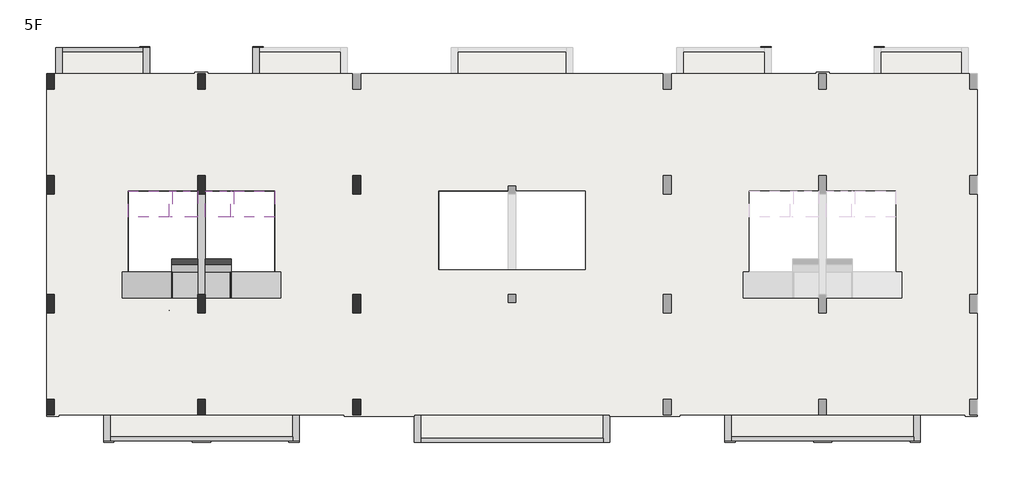
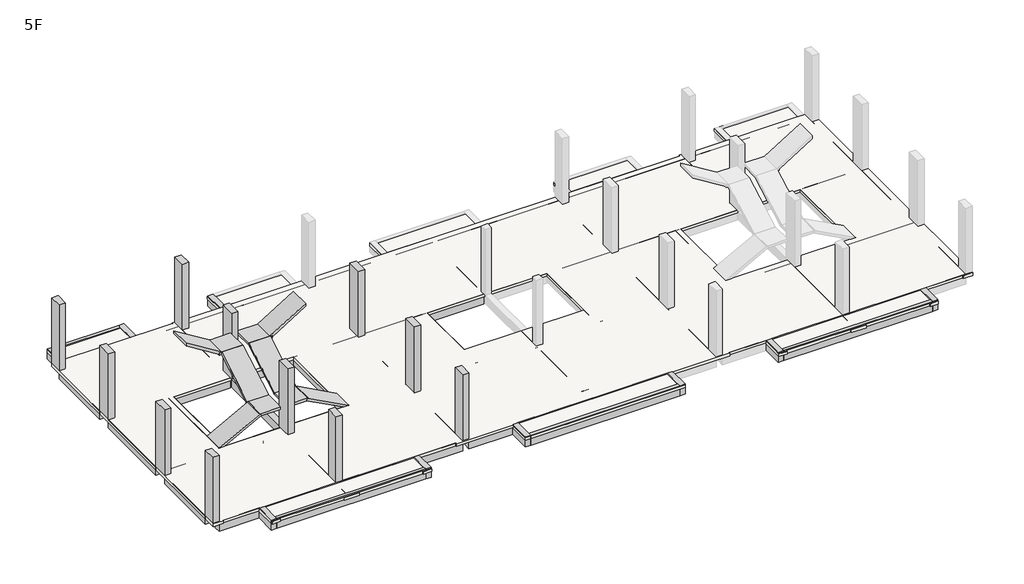
# One storey, part 1 of 2: 48 beams, 11 columns, 2 slabs.
"""IFC4 building model written with IfcOpenShell, lengths in millimetres."""

from ifc_helpers import new_model, si_unit, frame, origin, place, context, project, spatial, polyline, outline, extrude, faceted_brep, element, save

model = new_model("IFC4")

# Units and contexts
model_context = context("Model", 3, world=origin())
ifc_project = project(units=[si_unit("LENGTHUNIT", "METRE", prefix="MILLI")], contexts=[model_context])

# Site, building, storey
site = spatial("IfcSite", under=ifc_project)
building = spatial("IfcBuilding", under=site)
storey = spatial("IfcBuildingStorey", under=building, Name="5F", Elevation=13930.0)

# Beams
placement = place(None, origin())
element("IfcBeam", 1, ObjectType="M_Concrete-Rectangular Beam : 1000x120", at=placement, inside=storey, context=model_context, shape_type="Brep", body=[
    faceted_brep([(4730.4772067, 5424.9999998, 14980.0), (4730.4772067, 4424.9999998, 14980.0), (4787.1330577, 4424.9999998, 14874.2166623), (4787.1330577, 5424.9999998, 14874.2166623), (4700.0000007, 5424.9999998, 14963.6768996), (2770.0, 5424.9999998, 13930.0), (2770.0, 4424.9999998, 13930.0), (4700.0000007, 4424.9999998, 14963.6768996), (3024.1661582, 4424.9999998, 13930.0), (4760.5888269, 4424.9999998, 14860.0), (3024.1661582, 4449.9999998, 13930.0), (3020.0, 4449.9999998, 13927.7686728), (3020.0, 5424.9999998, 13927.7686728), (4760.5888269, 5424.9999998, 14860.0), (3020.0, 5424.9999998, 13930.0), (3020.0, 4449.9999998, 13930.0)], [[[0, 1, 2, 3]], [[1, 0, 4, 5, 6, 7]], [[2, 1, 7, 6, 8, 9]], [[3, 2, 9, 8, 10, 11, 12, 13]], [[0, 3, 13, 12, 14, 5, 4]], [[5, 14, 15, 10, 8, 6]], [[14, 12, 11, 15]], [[10, 15, 11]]]),
])
element("IfcBeam", 2, ObjectType="M_Concrete-Rectangular Beam : 1000x120", at=placement, inside=storey, context=model_context, shape_type="Brep", body=[
    faceted_brep([(4700.0000007, 7550.0000002, 16180.0), (5700.0000007, 7550.0000002, 16180.0), (5700.0000007, 7609.0063595, 16075.5095719), (4700.0000007, 7609.0063595, 16075.5095719), (4700.0000007, 5424.9999998, 14980.0), (4700.0000007, 5484.0063591, 14875.5095719), (5700.0000007, 5484.0063591, 14875.5095719), (5700.0000007, 5424.9999998, 14980.0), (5700.0000007, 5524.9999998, 14898.6589219), (5700.0000007, 7581.5414925, 16060.0), (4700.0000007, 5524.9999998, 14898.6589219), (4700.0000007, 7581.5414925, 16060.0)], [[[0, 1, 2, 3]], [[4, 5, 6, 7]], [[1, 0, 4, 7]], [[2, 1, 7, 6, 8, 9]], [[3, 2, 9, 8, 6, 5, 10, 11]], [[0, 3, 11, 10, 5, 4]]]),
])
element("IfcBeam", 3, ObjectType="M_Concrete-Rectangular Beam : 1000x120", at=placement, inside=storey, context=model_context, shape_type="Brep", body=[
    faceted_brep([(4600.0000007, 7550.0000002, 16180.0), (4600.0000007, 8550.0000002, 16180.0), (4600.0000007, 8550.0000002, 16060.0), (4600.0000007, 7550.0000002, 16060.0), (5700.0000007, 8550.0000002, 16060.0), (5700.0000007, 8550.0000002, 16180.0), (5700.0000007, 7550.0000002, 16180.0), (5700.0000007, 7609.0063595, 16075.5095719), (5700.0000007, 7581.5414925, 16060.0), (4700.0000007, 7550.0000002, 16180.0), (4700.0000007, 7581.5414925, 16060.0), (4700.0000007, 7550.0000002, 16060.0), (4700.0000007, 7609.0063595, 16075.5095719)], [[[0, 1, 2, 3]], [[4, 5, 6, 7, 8]], [[1, 0, 9, 6, 5]], [[2, 1, 5, 4]], [[3, 2, 4, 8, 10, 11]], [[0, 3, 11, 9]], [[12, 7, 6, 9]], [[7, 12, 10, 8]], [[12, 9, 11, 10]]]),
])
element("IfcBeam", 4, ObjectType="M_Concrete-Rectangular Beam : 1000x120", at=placement, inside=storey, context=model_context, shape_type="Brep", body=[
    faceted_brep([(3019.99996, 7549.9999993, 17230.0), (4715.7503089, 7549.9999993, 16180.0), (4715.7503089, 8549.9999993, 16180.0), (3019.99996, 8549.9999993, 17230.0), (4600.0000007, 8549.9999993, 16180.0), (4600.0000007, 8549.9999993, 16110.5302519), (3020.0, 8549.9999993, 17088.8582245), (4600.0000007, 7549.9999993, 16110.5302519), (3020.0, 7549.9999993, 17088.8582245), (4600.0000007, 7549.9999993, 16180.0), (4700.0000007, 7549.9999993, 16180.0)], [[[0, 1, 2, 3]], [[3, 2, 4, 5, 6]], [[5, 7, 8, 6]], [[1, 0, 8, 7, 9, 10]], [[4, 9, 7, 5]], [[9, 4, 2, 1, 10]], [[0, 3, 6, 8]]]),
])
element("IfcBeam", 5, ObjectType="M_Concrete-Rectangular Beam : 1000x120", at=placement, inside=storey, context=model_context, shape_type="Brep", body=[
    faceted_brep([(5700.0000007, 5524.9999998, 14860.0), (4700.0000007, 5524.9999998, 14860.0), (4700.0000007, 5524.9999998, 14898.6589219), (5700.0000007, 5524.9999998, 14898.6589219), (5700.0000007, 4424.9999998, 14860.0), (5700.0000007, 4424.9999998, 14980.0), (4730.4772067, 4424.9999998, 14980.0), (4787.1330577, 4424.9999998, 14874.2166623), (4760.5888269, 4424.9999998, 14860.0), (5700.0000007, 5424.9999998, 14980.0), (4700.0000007, 5424.9999998, 14980.0), (4700.0000007, 4424.9999998, 14980.0), (5700.0000007, 5484.0063591, 14875.5095719), (4760.5888269, 5424.9999998, 14860.0), (4700.0000007, 5424.9999998, 14860.0), (4700.0000007, 4424.9999998, 14963.6768996), (4700.0000007, 5484.0063591, 14875.5095719), (4700.0000007, 5424.9999998, 14963.6768996), (4730.4772067, 5424.9999998, 14980.0), (4787.1330577, 5424.9999998, 14874.2166623)], [[[0, 1, 2, 3]], [[4, 5, 6, 7, 8]], [[6, 5, 9, 10, 11]], [[5, 4, 0, 3, 12, 9]], [[1, 0, 4, 8, 13, 14]], [[15, 11, 10, 16, 2, 1, 14, 17]], [[6, 18, 19, 7]], [[18, 6, 15, 17]], [[7, 19, 13, 8]], [[19, 18, 17, 14, 13]], [[11, 15, 6]], [[12, 16, 10, 9]], [[16, 12, 3, 2]]]),
])
element("IfcBeam", 6, ObjectType="M_Concrete-Rectangular Beam : 1000x120", at=placement, inside=storey, context=model_context, shape_type="Brep", body=[
    faceted_brep([(6969.5227948, 4424.9999998, 14980.0), (6969.5227948, 5424.9999998, 14980.0), (6912.8669437, 5424.9999998, 14874.2166623), (6912.8669437, 4424.9999998, 14874.2166623), (7000.0000007, 4424.9999998, 14963.6768996), (8930.0000014, 4424.9999998, 13930.0), (8930.0000014, 5424.9999998, 13930.0), (7000.0000007, 5424.9999998, 14963.6768996), (6939.4111745, 4424.9999998, 14860.0), (8675.8338433, 4424.9999998, 13930.0), (6939.4111745, 5424.9999998, 14860.0), (8680.0, 5424.9999998, 13927.7686736), (8680.0, 4449.9999998, 13927.7686736), (8675.8338433, 4449.9999998, 13930.0), (8680.0, 5424.9999998, 13930.0), (8680.0, 4449.9999998, 13930.0)], [[[0, 1, 2, 3]], [[1, 0, 4, 5, 6, 7]], [[0, 3, 8, 9, 5, 4]], [[3, 2, 10, 11, 12, 13, 9, 8]], [[2, 1, 7, 6, 14, 11, 10]], [[9, 13, 15, 14, 6, 5]], [[11, 14, 15, 12]], [[15, 13, 12]]]),
])
element("IfcBeam", 7, ObjectType="M_Concrete-Rectangular Beam : 1000x120", at=placement, inside=storey, context=model_context, shape_type="Brep", body=[
    faceted_brep([(7000.0000007, 7550.0000002, 16180.0), (7000.0000007, 7609.0063595, 16075.5095719), (6000.0000007, 7609.0063595, 16075.5095719), (6000.0000007, 7550.0000002, 16180.0), (7000.0000007, 5424.9999998, 14980.0), (6000.0000007, 5424.9999998, 14980.0), (6000.0000007, 5484.0063591, 14875.5095719), (7000.0000007, 5484.0063591, 14875.5095719), (6000.0000007, 7581.5414925, 16060.0), (6000.0000007, 5524.9999998, 14898.6589219), (7000.0000007, 7581.5414925, 16060.0), (7000.0000007, 5524.9999998, 14898.6589219)], [[[0, 1, 2, 3]], [[4, 5, 6, 7]], [[3, 5, 4, 0]], [[2, 8, 9, 6, 5, 3]], [[1, 10, 11, 7, 6, 9, 8, 2]], [[0, 4, 7, 11, 10, 1]]]),
])
element("IfcBeam", 8, ObjectType="M_Concrete-Rectangular Beam : 1000x120", at=placement, inside=storey, context=model_context, shape_type="Brep", body=[
    faceted_brep([(7100.0000007, 8550.0000002, 16180.0), (7100.0000007, 7550.0000002, 16180.0), (7100.0000007, 7550.0000002, 16060.0), (7100.0000007, 8550.0000002, 16060.0), (6000.0000007, 8550.0000002, 16180.0), (6000.0000007, 8550.0000002, 16060.0), (6000.0000007, 7581.5414925, 16060.0), (6000.0000007, 7609.0063595, 16075.5095719), (6000.0000007, 7550.0000002, 16180.0), (7000.0000007, 7550.0000002, 16180.0), (7000.0000007, 7550.0000002, 16060.0), (7000.0000007, 7581.5414925, 16060.0), (7000.0000007, 7609.0063595, 16075.5095719)], [[[0, 1, 2, 3]], [[4, 5, 6, 7, 8]], [[1, 0, 4, 8, 9]], [[0, 3, 5, 4]], [[3, 2, 10, 11, 6, 5]], [[2, 1, 9, 10]], [[12, 9, 8, 7]], [[12, 7, 6, 11]], [[9, 12, 11, 10]]]),
])
element("IfcBeam", 9, ObjectType="M_Concrete-Rectangular Beam : 1000x120", at=placement, inside=storey, context=model_context, shape_type="Brep", body=[
    faceted_brep([(6984.2496926, 7549.9999993, 16180.0), (8680.0000414, 7549.9999993, 17230.0), (8680.0, 8549.9999993, 17229.9999744), (6984.2496926, 8549.9999993, 16180.0), (8680.0, 8549.9999993, 17088.8582236), (7100.0000007, 8549.9999993, 16110.5302519), (7100.0000007, 8549.9999993, 16180.0), (7100.0000007, 7549.9999993, 16110.5302519), (8680.0, 7549.9999993, 17088.8582236), (7000.0000007, 7549.9999993, 16180.0), (7100.0000007, 7549.9999993, 16180.0)], [[[0, 1, 2, 3]], [[3, 2, 4, 5, 6]], [[7, 5, 4, 8]], [[1, 0, 9, 10, 7, 8]], [[10, 6, 5, 7]], [[6, 10, 9, 0, 3]], [[2, 1, 8, 4]]]),
])
element("IfcBeam", 10, ObjectType="M_Concrete-Rectangular Beam : 1000x120", at=placement, inside=storey, context=model_context, shape_type="Brep", body=[
    faceted_brep([(7000.0000007, 5524.9999998, 14860.0), (6000.0000007, 5524.9999998, 14860.0), (6000.0000007, 5524.9999998, 14898.6589219), (7000.0000007, 5524.9999998, 14898.6589219), (6000.0000007, 4424.9999998, 14980.0), (6000.0000007, 4424.9999998, 14860.0), (6939.4111745, 4424.9999998, 14860.0), (6912.8669437, 4424.9999998, 14874.2166623), (6969.5227948, 4424.9999998, 14980.0), (7000.0000007, 4424.9999998, 14980.0), (7000.0000007, 5424.9999998, 14980.0), (6000.0000007, 5424.9999998, 14980.0), (6000.0000007, 5484.0063591, 14875.5095719), (7000.0000007, 5424.9999998, 14860.0), (6939.4111745, 5424.9999998, 14860.0), (7000.0000007, 4424.9999998, 14963.6768996), (7000.0000007, 5424.9999998, 14963.6768996), (7000.0000007, 5484.0063591, 14875.5095719), (6969.5227948, 5424.9999998, 14980.0), (6912.8669437, 5424.9999998, 14874.2166623)], [[[0, 1, 2, 3]], [[4, 5, 6, 7, 8]], [[8, 9, 10, 11, 4]], [[5, 4, 11, 12, 2, 1]], [[1, 0, 13, 14, 6, 5]], [[9, 15, 16, 13, 0, 3, 17, 10]], [[18, 8, 7, 19]], [[8, 18, 16, 15]], [[19, 7, 6, 14]], [[18, 19, 14, 13, 16]], [[15, 9, 8]], [[17, 12, 11, 10]], [[12, 17, 3, 2]]]),
])
element("IfcBeam", 11, ObjectType="M_Concrete-Rectangular Beam : 150x500", at=placement, inside=storey, context=model_context, shape_type="SweptSolid", body=[
    extrude(outline(polyline([(2320.0000398, -1099.9999999), (2320.0000398, -949.9999999), (9380.0000399, -949.9999999), (9380.0000399, -1099.9999999), (2320.0000398, -1099.9999999)])), frame((0.0, 0.0, 13430.0), z_axis=(0.0, 0.0, 1.0), x_axis=(1.0, 0.0, 0.0)), (0.0, 0.0, 1.0), 500.0),
])
element("IfcBeam", 12, ObjectType="M_Concrete-Rectangular Beam : 150x500", at=placement, inside=storey, context=model_context, shape_type="SweptSolid", body=[
    extrude(outline(polyline([(26320.012858, -1100.2407813), (26320.012858, -950.2407813), (33380.0128581, -950.2407813), (33380.0128581, -1100.2407813), (26320.012858, -1100.2407813)])), frame((0.0, 0.0, 13430.0), z_axis=(0.0, 0.0, 1.0), x_axis=(1.0, 0.0, 0.0)), (0.0, 0.0, 1.0), 500.0),
])
element("IfcBeam", 13, ObjectType="M_Concrete-Rectangular Beam : 150x500", at=placement, inside=storey, context=model_context, shape_type="SweptSolid", body=[
    extrude(outline(polyline([(14320.0998335, -1150.2407813), (14320.0998335, -1000.2407813), (21380.0998336, -1000.2407813), (21380.0998336, -1150.2407813), (14320.0998335, -1150.2407813)])), frame((0.0, 0.0, 13430.0), z_axis=(0.0, 0.0, 1.0), x_axis=(1.0, 0.0, 0.0)), (0.0, 0.0, 1.0), 500.0),
])
element("IfcBeam", 14, ObjectType="M_Concrete-Rectangular Beam : 150x500", at=placement, inside=storey, context=model_context, shape_type="SweptSolid", body=[
    extrude(outline(polyline([(3609.9999642, 14100.0000002), (3609.9999642, 13950.0000002), (475.0000398, 13950.0000002), (475.0000398, 14100.0000002), (3609.9999642, 14100.0000002)])), frame((0.0, 0.0, 13430.0), z_axis=(0.0, 0.0, 1.0), x_axis=(1.0, 0.0, 0.0)), (0.0, 0.0, 1.0), 500.0),
])
element("IfcBeam", 15, ObjectType="M_Concrete-Rectangular Beam : 250x400", at=placement, inside=storey, context=model_context, shape_type="Brep", body=[
    faceted_brep([(8930.0, 8549.9999993, 13930.0), (8680.0, 8549.9999993, 13930.0), (8680.0, 5424.9999998, 13930.0), (8680.0, 4449.9999998, 13930.0), (8930.0, 4449.9999998, 13930.0), (8680.0, 8549.9999993, 13788.8582236), (8680.0, 8549.9999993, 13530.0), (8680.0, 4449.9999998, 13530.0), (8680.0, 4449.9999998, 13927.7686736), (8930.0, 8549.9999993, 13530.0), (8930.0, 4449.9999998, 13530.0)], [[[0, 1, 2, 3, 4]], [[1, 5, 6, 7, 8, 3, 2]], [[6, 9, 10, 7]], [[9, 0, 4, 10]], [[1, 0, 9, 6, 5]], [[4, 3, 8, 7, 10]]]),
])
element("IfcBeam", 16, ObjectType="M_Concrete-Rectangular Beam : 250x400", at=placement, inside=storey, context=model_context, shape_type="Brep", body=[
    faceted_brep([(15020.0000057, 8549.9999993, 13930.0), (14770.0000057, 8549.9999993, 13930.0), (14770.0000057, 4449.9999998, 13930.0), (15020.0000057, 4449.9999998, 13930.0), (15020.0000057, 8549.9999993, 13530.0), (15020.0000057, 8549.9999993, 13788.8582241), (15020.0000057, 4449.9999998, 13530.0), (14770.0000057, 8549.9999993, 13530.0), (14770.0000057, 4449.9999998, 13530.0)], [[[0, 1, 2, 3]], [[4, 5, 0, 3, 6]], [[7, 4, 6, 8]], [[1, 7, 8, 2]], [[1, 0, 5, 4, 7]], [[3, 2, 8, 6]]]),
])
element("IfcBeam", 17, ObjectType="M_Concrete-Rectangular Beam : 250x400", at=placement, inside=storey, context=model_context, shape_type="Brep", body=[
    faceted_brep([(3020.0, 8549.9999993, 13930.0), (2770.0, 8549.9999993, 13930.0), (2770.0, 4449.9999998, 13930.0), (3020.0, 4449.9999998, 13930.0), (3020.0, 5424.9999998, 13930.0), (3020.0, 8549.9999993, 13530.0), (3020.0, 8549.9999993, 13788.8582245), (3020.0, 4449.9999998, 13927.7686728), (3020.0, 4449.9999998, 13530.0), (2770.0, 8549.9999993, 13530.0), (2770.0, 4449.9999998, 13530.0)], [[[0, 1, 2, 3, 4]], [[5, 6, 0, 4, 3, 7, 8]], [[9, 5, 8, 10]], [[1, 9, 10, 2]], [[1, 0, 6, 5, 9]], [[3, 2, 10, 8, 7]]]),
])
element("IfcBeam", 18, ObjectType="M_Concrete-Rectangular Beam : 250x500", at=placement, inside=storey, context=model_context, shape_type="Brep", body=[
    faceted_brep([(225.0000398, 13101.5853605, 13930.0), (225.0000398, 13101.5853605, 13430.0), (475.0000398, 13101.5853605, 13430.0), (475.0000398, 13101.5853605, 13930.0), (475.0000398, 13950.0000002, 13930.0), (475.0000398, 14100.0000002, 13930.0), (225.0000398, 14100.0000002, 13930.0), (475.0000398, 13950.0000002, 13430.0), (475.0000398, 14100.0000002, 13430.0), (225.0000398, 14100.0000002, 13430.0)], [[[0, 1, 2, 3]], [[0, 3, 4, 5, 6]], [[3, 2, 7, 8, 5, 4]], [[2, 1, 9, 8, 7]], [[1, 0, 6, 9]], [[6, 5, 8, 9]]]),
])
element("IfcBeam", 19, ObjectType="M_Concrete-Rectangular Beam : 250x500", at=placement, inside=storey, context=model_context, shape_type="Brep", body=[
    faceted_brep([(2070.0000398, -1099.9999999, 13930.0), (2320.0000398, -1099.9999999, 13930.0), (2320.0000398, -949.9999999, 13930.0), (2320.0000398, -100.0000007, 13930.0), (2070.0000398, -100.0000007, 13930.0), (2320.0000398, -1099.9999999, 13430.0), (2320.0000398, -949.9999999, 13430.0), (2320.0000398, -100.0000007, 13430.0), (2070.0000398, -1099.9999999, 13430.0), (2070.0000398, -100.0000007, 13430.0)], [[[0, 1, 2, 3, 4]], [[1, 5, 6, 7, 3, 2]], [[5, 8, 9, 7, 6]], [[8, 0, 4, 9]], [[4, 3, 7, 9]], [[1, 0, 8, 5]]]),
])
element("IfcBeam", 20, ObjectType="M_Concrete-Rectangular Beam : 250x500", at=placement, inside=storey, context=model_context, shape_type="Brep", body=[
    faceted_brep([(9380.0000399, -1099.9999999, 13930.0), (9630.0000399, -1099.9999999, 13930.0), (9630.0000399, -100.0000007, 13930.0), (9380.0000399, -100.0000007, 13930.0), (9380.0000399, -949.9999999, 13930.0), (9380.0000399, -1099.9999999, 13430.0), (9380.0000399, -100.0000007, 13430.0), (9380.0000399, -949.9999999, 13430.0), (9630.0000399, -1099.9999999, 13430.0), (9630.0000399, -100.0000007, 13430.0)], [[[0, 1, 2, 3, 4]], [[5, 0, 4, 3, 6, 7]], [[8, 5, 7, 6, 9]], [[1, 8, 9, 2]], [[1, 0, 5, 8]], [[3, 2, 9, 6]]]),
])
element("IfcBeam", 21, ObjectType="M_Concrete-Rectangular Beam : 250x500", at=placement, inside=storey, context=model_context, shape_type="Brep", body=[
    faceted_brep([(26070.012858, -1100.2407813, 13930.0), (26320.012858, -1100.2407813, 13930.0), (26320.012858, -950.2407813, 13930.0), (26320.012858, -100.0000013, 13930.0), (26070.012858, -100.0000013, 13930.0), (26320.012858, -1100.2407813, 13430.0), (26320.012858, -950.2407813, 13430.0), (26320.012858, -100.0000013, 13430.0), (26070.012858, -1100.2407813, 13430.0), (26070.012858, -100.0000013, 13430.0)], [[[0, 1, 2, 3, 4]], [[1, 5, 6, 7, 3, 2]], [[5, 8, 9, 7, 6]], [[8, 0, 4, 9]], [[1, 0, 8, 5]], [[4, 3, 7, 9]]]),
])
element("IfcBeam", 22, ObjectType="M_Concrete-Rectangular Beam : 250x500", at=placement, inside=storey, context=model_context, shape_type="Brep", body=[
    faceted_brep([(33380.0128581, -1100.2407813, 13930.0), (33630.0128581, -1100.2407813, 13930.0), (33630.0128581, -100.0000013, 13930.0), (33380.0128581, -100.0000013, 13930.0), (33380.0128581, -950.2407813, 13930.0), (33380.0128581, -1100.2407813, 13430.0), (33380.0128581, -100.0000013, 13430.0), (33380.0128581, -950.2407813, 13430.0), (33630.0128581, -1100.2407813, 13430.0), (33630.0128581, -100.0000013, 13430.0)], [[[0, 1, 2, 3, 4]], [[5, 0, 4, 3, 6, 7]], [[8, 5, 7, 6, 9]], [[1, 8, 9, 2]], [[1, 0, 5, 8]], [[3, 2, 9, 6]]]),
])
element("IfcBeam", 23, ObjectType="M_Concrete-Rectangular Beam : 250x500", at=placement, inside=storey, context=model_context, shape_type="Brep", body=[
    faceted_brep([(14070.0998335, -1150.2407813, 13930.0), (14320.0998335, -1150.2407813, 13930.0), (14320.0998335, -1000.2407813, 13930.0), (14320.0998335, -100.0000007, 13930.0), (14070.0998335, -100.0000007, 13930.0), (14320.0998335, -1150.2407813, 13430.0), (14320.0998335, -1000.2407813, 13430.0), (14320.0998335, -100.0000007, 13430.0), (14070.0998335, -1150.2407813, 13430.0), (14070.0998335, -100.0000007, 13430.0)], [[[0, 1, 2, 3, 4]], [[1, 5, 6, 7, 3, 2]], [[5, 8, 9, 7, 6]], [[8, 0, 4, 9]], [[4, 3, 7, 9]], [[1, 0, 8, 5]]]),
])
element("IfcBeam", 24, ObjectType="M_Concrete-Rectangular Beam : 250x500", at=placement, inside=storey, context=model_context, shape_type="Brep", body=[
    faceted_brep([(21380.0998336, -1150.2407813, 13930.0), (21630.0998336, -1150.2407813, 13930.0), (21630.0998336, -100.0000007, 13930.0), (21380.0998336, -100.0000007, 13930.0), (21380.0998336, -1000.2407813, 13930.0), (21380.0998336, -1150.2407813, 13430.0), (21380.0998336, -100.0000007, 13430.0), (21380.0998336, -1000.2407813, 13430.0), (21630.0998336, -1150.2407813, 13430.0), (21630.0998336, -100.0000007, 13430.0)], [[[0, 1, 2, 3, 4]], [[5, 0, 4, 3, 6, 7]], [[8, 5, 7, 6, 9]], [[1, 8, 9, 2]], [[3, 2, 9, 6]], [[1, 0, 5, 8]]]),
])
element("IfcBeam", 25, ObjectType="M_Concrete-Rectangular Beam : 250x500", at=placement, inside=storey, context=model_context, shape_type="Brep", body=[
    faceted_brep([(8090.0434249, 14100.0000002, 13930.0), (7840.0434249, 14100.0000002, 13930.0), (7840.0434249, 13100.0000001, 13930.0), (8090.0434249, 13100.0000001, 13930.0), (8090.0434249, 13950.0000002, 13930.0), (7840.0434249, 14100.0000002, 13430.0), (7840.0434249, 13100.0000001, 13430.0), (8090.0434249, 14100.0000002, 13430.0), (8090.0434249, 13950.0000002, 13430.0), (8090.0434249, 13100.0000001, 13430.0)], [[[0, 1, 2, 3, 4]], [[1, 5, 6, 2]], [[5, 7, 8, 9, 6]], [[7, 0, 4, 3, 9, 8]], [[3, 2, 6, 9]], [[1, 0, 7, 5]]]),
])
element("IfcBeam", 26, ObjectType="M_Concrete-Rectangular Beam : 250x500", at=placement, inside=storey, context=model_context, shape_type="Brep", body=[
    faceted_brep([(3859.9999642, 14100.0000002, 13930.0), (3609.9999642, 14100.0000002, 13930.0), (3609.9999642, 13950.0000002, 13930.0), (3609.9999642, 13100.0000001, 13930.0), (3859.9999642, 13100.0000001, 13930.0), (3859.9999642, 14100.0000002, 13430.0), (3859.9999642, 13100.0000001, 13430.0), (3609.9999642, 14100.0000002, 13430.0), (3609.9999642, 13100.0000001, 13430.0), (3609.9999642, 13950.0000002, 13430.0)], [[[0, 1, 2, 3, 4]], [[5, 0, 4, 6]], [[7, 5, 6, 8, 9]], [[1, 7, 9, 8, 3, 2]], [[4, 3, 8, 6]], [[1, 0, 5, 7]]]),
])
element("IfcBeam", 27, ObjectType="M_Concrete-Rectangular Beam : 300x400", at=placement, inside=storey, context=model_context, shape_type="SweptSolid", body=[
    extrude(outline(polyline([(165.0, 9150.0000002), (-135.0, 9150.0000002), (-135.0, 12500.0000005), (165.0, 12500.0000005), (165.0, 9150.0000002)])), frame((0.0, 0.0, 13530.0), z_axis=(0.0, 0.0, 1.0), x_axis=(1.0, 0.0, 0.0)), (0.0, 0.0, 1.0), 400.0),
])
element("IfcBeam", 28, ObjectType="M_Concrete-Rectangular Beam : 300x400", at=placement, inside=storey, context=model_context, shape_type="SweptSolid", body=[
    extrude(outline(polyline([(165.0, 4550.0000002), (-135.0, 4550.0000002), (-135.0, 8450.0000002), (165.0, 8450.0000002), (165.0, 4550.0000002)])), frame((0.0, 0.0, 13530.0), z_axis=(0.0, 0.0, 1.0), x_axis=(1.0, 0.0, 0.0)), (0.0, 0.0, 1.0), 400.0),
])
element("IfcBeam", 29, ObjectType="M_Concrete-Rectangular Beam : 300x400", at=placement, inside=storey, context=model_context, shape_type="SweptSolid", body=[
    extrude(outline(polyline([(165.0, 500.0), (-135.0, 500.0), (-135.0, 3850.0000002), (165.0, 3850.0000002), (165.0, 500.0)])), frame((0.0, 0.0, 13530.0), z_axis=(0.0, 0.0, 1.0), x_axis=(1.0, 0.0, 0.0)), (0.0, 0.0, 1.0), 400.0),
])
element("IfcBeam", 30, ObjectType="M_Concrete-Rectangular Beam : 300x400", at=placement, inside=storey, context=model_context, shape_type="SweptSolid", body=[
    extrude(outline(polyline([(12000.0000027, 4550.0000002), (11700.0000027, 4550.0000002), (11700.0000027, 8450.0000002), (12000.0000027, 8450.0000002), (12000.0000027, 4550.0000002)])), frame((0.0, 0.0, 13530.0), z_axis=(0.0, 0.0, 1.0), x_axis=(1.0, 0.0, 0.0)), (0.0, 0.0, 1.0), 400.0),
])
element("IfcBeam", 31, ObjectType="M_Concrete-Rectangular Beam : 300x400", at=placement, inside=storey, context=model_context, shape_type="SweptSolid", body=[
    extrude(outline(polyline([(6000.0, 4550.0000002), (5700.0, 4550.0000002), (5700.0, 8450.0000002), (6000.0, 8450.0000002), (6000.0, 4550.0000002)])), frame((0.0, 0.0, 13530.0), z_axis=(0.0, 0.0, 1.0), x_axis=(1.0, 0.0, 0.0)), (0.0, 0.0, 1.0), 400.0),
])
element("IfcBeam", 32, ObjectType="M_Concrete-Rectangular Beam : 300x400", at=placement, inside=storey, context=model_context, shape_type="SweptSolid", body=[
    extrude(outline(polyline([(6000.0000007, 500.0), (5700.0000007, 500.0), (5700.0000007, 3850.0000002), (6000.0000007, 3850.0000002), (6000.0000007, 500.0)])), frame((0.0, 0.0, 13530.0), z_axis=(0.0, 0.0, 1.0), x_axis=(1.0, 0.0, 0.0)), (0.0, 0.0, 1.0), 400.0),
])
element("IfcBeam", 33, ObjectType="M_Concrete-Rectangular Beam : 300x400", at=placement, inside=storey, context=model_context, shape_type="SweptSolid", body=[
    extrude(outline(polyline([(6000.0000007, 9150.0000002), (5700.0000007, 9150.0000002), (5700.0000007, 12500.0000005), (6000.0000007, 12500.0000005), (6000.0000007, 9150.0000002)])), frame((0.0, 0.0, 13530.0), z_axis=(0.0, 0.0, 1.0), x_axis=(1.0, 0.0, 0.0)), (0.0, 0.0, 1.0), 400.0),
])
element("IfcBeam", 34, ObjectType="M_Concrete-Rectangular Beam : 300x400", at=placement, inside=storey, context=model_context, shape_type="SweptSolid", body=[
    extrude(outline(polyline([(12000.0000034, 500.0), (11700.0000034, 500.0), (11700.0000034, 3850.0000002), (12000.0000034, 3850.0000002), (12000.0000034, 500.0)])), frame((0.0, 0.0, 13530.0), z_axis=(0.0, 0.0, 1.0), x_axis=(1.0, 0.0, 0.0)), (0.0, 0.0, 1.0), 400.0),
])
element("IfcBeam", 35, ObjectType="M_Concrete-Rectangular Beam : 300x400", at=placement, inside=storey, context=model_context, shape_type="SweptSolid", body=[
    extrude(outline(polyline([(12000.0000034, 9150.0000002), (11700.0000034, 9150.0000002), (11700.0000034, 12500.0000005), (12000.0000034, 12500.0000005), (12000.0000034, 9150.0000002)])), frame((0.0, 0.0, 13530.0), z_axis=(0.0, 0.0, 1.0), x_axis=(1.0, 0.0, 0.0)), (0.0, 0.0, 1.0), 400.0),
])
element("IfcBeam", 36, ObjectType="M_Concrete-Rectangular Beam : 300x400", at=placement, inside=storey, context=model_context, shape_type="Brep", body=[
    faceted_brep([(6000.0000007, -100.0, 13880.0), (5700.0000007, -100.0000007, 13880.0), (5700.0000007, -949.9999999, 13880.0), (6000.0000007, -949.9999999, 13880.0), (6000.0000007, -949.9999999, 13480.0), (6000.0000007, -100.0, 13480.0), (5700.0000007, -100.0000007, 13480.0), (5700.0000007, -949.9999999, 13480.0)], [[[0, 1, 2, 3]], [[3, 4, 5, 0]], [[6, 5, 4, 7]], [[1, 6, 7, 2]], [[0, 5, 6, 1]], [[3, 2, 7, 4]]]),
])
element("IfcBeam", 37, ObjectType="M_Concrete-Rectangular Beam : 300x400", at=placement, inside=storey, context=model_context, shape_type="Brep", body=[
    faceted_brep([(18000.0064311, -100.0, 13880.0), (17700.0064311, -100.0000007, 13880.0), (17700.0064311, -1000.2407813, 13880.0), (18000.0064311, -1000.2407813, 13880.0), (18000.0064311, -1000.2407813, 13480.0), (18000.0064311, -100.0, 13480.0), (17700.0064311, -100.0000007, 13480.0), (17700.0064311, -1000.2407813, 13480.0)], [[[0, 1, 2, 3]], [[3, 4, 5, 0]], [[6, 5, 4, 7]], [[1, 6, 7, 2]], [[0, 5, 6, 1]], [[3, 2, 7, 4]]]),
])
element("IfcBeam", 38, ObjectType="M_Concrete-Rectangular Beam : 300x400", at=placement, inside=storey, context=model_context, shape_type="Brep", body=[
    faceted_brep([(30000.0064292, -100.0, 13880.0), (29700.0064292, -100.0000013, 13880.0), (29700.0064292, -950.2407813, 13880.0), (30000.0064292, -950.2407813, 13880.0), (30000.0064292, -950.2407813, 13480.0), (30000.0064292, -100.0, 13480.0), (29700.0064292, -100.0000013, 13480.0), (29700.0064292, -950.2407813, 13480.0)], [[[0, 1, 2, 3]], [[3, 4, 5, 0]], [[6, 5, 4, 7]], [[1, 6, 7, 2]], [[0, 5, 6, 1]], [[3, 2, 7, 4]]]),
])
element("IfcBeam", 39, ObjectType="M_Concrete-Rectangular Beam : 300x500", at=placement, inside=storey, context=model_context, shape_type="Brep", body=[
    faceted_brep([(164.9999993, 13100.0000001, 13930.0), (164.9999993, 12800.0000001, 13930.0), (5700.0000007, 12800.0000001, 13930.0), (5700.0000007, 13100.0000001, 13930.0), (3859.9999642, 13100.0000001, 13930.0), (3609.9999642, 13100.0000001, 13930.0), (164.9999993, 12800.0000001, 13430.0), (5700.0000007, 12800.0000001, 13430.0), (164.9999993, 13100.0000001, 13430.0), (3609.9999642, 13100.0000001, 13430.0), (3859.9999642, 13100.0000001, 13430.0), (5700.0000007, 13100.0000001, 13430.0)], [[[0, 1, 2, 3, 4, 5]], [[1, 6, 7, 2]], [[6, 8, 9, 10, 11, 7]], [[8, 0, 5, 4, 3, 11, 10, 9]], [[1, 0, 8, 6]], [[3, 2, 7, 11]]]),
])
element("IfcBeam", 40, ObjectType="M_Concrete-Rectangular Beam : 300x500", at=placement, inside=storey, context=model_context, shape_type="Brep", body=[
    faceted_brep([(164.9649925, 8849.9999993, 13930.0), (164.9649925, 8549.9999993, 13930.0), (2770.0, 8549.9999993, 13930.0), (3020.0, 8549.9999993, 13930.0), (5699.9649933, 8549.9999993, 13930.0), (5699.9649933, 8849.9999993, 13930.0), (164.9649925, 8549.9999993, 13430.0), (5699.9649933, 8549.9999993, 13430.0), (164.9649925, 8849.9999993, 13430.0), (5699.9649933, 8849.9999993, 13430.0)], [[[0, 1, 2, 3, 4, 5]], [[1, 6, 7, 4, 3, 2]], [[6, 8, 9, 7]], [[8, 0, 5, 9]], [[1, 0, 8, 6]], [[5, 4, 7, 9]]]),
])
element("IfcBeam", 41, ObjectType="M_Concrete-Rectangular Beam : 300x500", at=placement, inside=storey, context=model_context, shape_type="Brep", body=[
    faceted_brep([(165.0, 4449.9999998, 13930.0), (165.0, 4149.9999998, 13930.0), (5700.0000007, 4149.9999998, 13930.0), (5700.0000007, 4449.9999998, 13930.0), (3024.1661582, 4449.9999998, 13930.0), (3020.0, 4449.9999998, 13930.0), (2770.0, 4449.9999998, 13930.0), (165.0, 4149.9999998, 13430.0), (5700.0000007, 4149.9999998, 13430.0), (165.0, 4449.9999998, 13430.0), (5700.0000007, 4449.9999998, 13430.0)], [[[0, 1, 2, 3, 4, 5, 6]], [[1, 7, 8, 2]], [[7, 9, 10, 8]], [[9, 0, 6, 5, 4, 3, 10]], [[1, 0, 9, 7]], [[3, 2, 8, 10]]]),
])
element("IfcBeam", 42, ObjectType="M_Concrete-Rectangular Beam : 300x500", at=placement, inside=storey, context=model_context, shape_type="Brep", body=[
    faceted_brep([(165.0, 199.9999993, 13930.0), (165.0, -100.0000007, 13930.0), (2070.0000398, -100.0000007, 13930.0), (2320.0000398, -100.0000007, 13930.0), (5700.0000007, -100.0000007, 13930.0), (5700.0000007, 199.9999993, 13930.0), (165.0, -100.0000007, 13430.0), (2070.0000398, -100.0000007, 13430.0), (2320.0000398, -100.0000007, 13430.0), (5700.0000007, -100.0000007, 13430.0), (165.0, 199.9999993, 13430.0), (5700.0000007, 199.9999993, 13430.0)], [[[0, 1, 2, 3, 4, 5]], [[1, 6, 7, 8, 9, 4, 3, 2]], [[6, 10, 11, 9, 8, 7]], [[10, 0, 5, 11]], [[1, 0, 10, 6]], [[5, 4, 9, 11]]]),
])
element("IfcBeam", 43, ObjectType="M_Concrete-Rectangular Beam : 300x500", at=placement, inside=storey, context=model_context, shape_type="Brep", body=[
    faceted_brep([(5999.9649933, 8849.9999993, 13930.0), (5999.9649933, 8549.9999993, 13930.0), (8680.0, 8549.9999993, 13930.0), (8930.0, 8549.9999993, 13930.0), (11699.964996, 8549.9999993, 13930.0), (11699.964996, 8849.9999993, 13930.0), (5999.9649933, 8549.9999993, 13430.0), (11699.964996, 8549.9999993, 13430.0), (5999.9649933, 8849.9999993, 13430.0), (11699.964996, 8849.9999993, 13430.0)], [[[0, 1, 2, 3, 4, 5]], [[1, 6, 7, 4, 3, 2]], [[6, 8, 9, 7]], [[8, 0, 5, 9]], [[1, 0, 8, 6]], [[5, 4, 7, 9]]]),
])
element("IfcBeam", 44, ObjectType="M_Concrete-Rectangular Beam : 300x500", at=placement, inside=storey, context=model_context, shape_type="Brep", body=[
    faceted_brep([(6000.0000007, 4449.9999998, 13930.0), (6000.0000007, 4149.9999998, 13930.0), (11700.0000034, 4149.9999998, 13930.0), (11700.0000034, 4449.9999998, 13930.0), (8930.0, 4449.9999998, 13930.0), (8680.0, 4449.9999998, 13930.0), (8675.8338433, 4449.9999998, 13930.0), (6000.0000007, 4149.9999998, 13430.0), (11700.0000034, 4149.9999998, 13430.0), (6000.0000007, 4449.9999998, 13430.0), (11700.0000034, 4449.9999998, 13430.0)], [[[0, 1, 2, 3, 4, 5, 6]], [[1, 7, 8, 2]], [[7, 9, 10, 8]], [[9, 0, 6, 5, 4, 3, 10]], [[1, 0, 9, 7]], [[3, 2, 8, 10]]]),
])
element("IfcBeam", 45, ObjectType="M_Concrete-Rectangular Beam : 300x500", at=placement, inside=storey, context=model_context, shape_type="Brep", body=[
    faceted_brep([(6000.0000007, 199.9999993, 13930.0), (6000.0000007, -100.0000007, 13930.0), (9380.0000399, -100.0000007, 13930.0), (9630.0000399, -100.0000007, 13930.0), (11700.0000034, -100.0000007, 13930.0), (11700.0000034, 199.9999993, 13930.0), (6000.0000007, -100.0000007, 13430.0), (9380.0000399, -100.0000007, 13430.0), (9630.0000399, -100.0000007, 13430.0), (11700.0000034, -100.0000007, 13430.0), (6000.0000007, 199.9999993, 13430.0), (11700.0000034, 199.9999993, 13430.0)], [[[0, 1, 2, 3, 4, 5]], [[1, 6, 7, 8, 9, 4, 3, 2]], [[6, 10, 11, 9, 8, 7]], [[10, 0, 5, 11]], [[1, 0, 10, 6]], [[5, 4, 9, 11]]]),
])
element("IfcBeam", 46, ObjectType="M_Concrete-Rectangular Beam : 300x500", at=placement, inside=storey, context=model_context, shape_type="Brep", body=[
    faceted_brep([(11999.964996, 8849.9999993, 13930.0), (12000.0000027, 8549.9999993, 13930.0), (14770.0000057, 8549.9999993, 13930.0), (15020.0000057, 8549.9999993, 13930.0), (17699.9649983, 8549.9999993, 13930.0), (17699.9649983, 8849.9999993, 13930.0), (11999.964996, 8549.9999993, 13430.0), (17699.9649983, 8549.9999993, 13430.0), (11999.964996, 8849.9999993, 13430.0), (17699.9649983, 8849.9999993, 13430.0)], [[[0, 1, 2, 3, 4, 5]], [[1, 6, 7, 4, 3, 2]], [[6, 8, 9, 7]], [[8, 0, 5, 9]], [[8, 6, 1, 0]], [[5, 4, 7, 9]]]),
])
element("IfcBeam", 47, ObjectType="M_Concrete-Rectangular Beam : 300x500", at=placement, inside=storey, context=model_context, shape_type="Brep", body=[
    faceted_brep([(12000.0000027, 4449.9999998, 13930.0), (12000.0000034, 4149.9999998, 13930.0), (17700.0000058, 4149.9999998, 13930.0), (17700.0000058, 4449.9999998, 13930.0), (15020.0000057, 4449.9999998, 13930.0), (14770.0000057, 4449.9999998, 13930.0), (12000.0000034, 4149.9999998, 13430.0), (17700.0000058, 4149.9999998, 13430.0), (12000.0000034, 4449.9999998, 13430.0), (17700.0000058, 4449.9999998, 13430.0)], [[[0, 1, 2, 3, 4, 5]], [[1, 6, 7, 2]], [[6, 8, 9, 7]], [[8, 0, 5, 4, 3, 9]], [[6, 1, 0, 8]], [[3, 2, 7, 9]]]),
])
element("IfcBeam", 48, ObjectType="M_Concrete-Rectangular Beam : 300x500", at=placement, inside=storey, context=model_context, shape_type="Brep", body=[
    faceted_brep([(12000.0000034, 199.9999993, 13930.0), (12000.0000034, -100.0000007, 13930.0), (14070.0998335, -100.0000007, 13930.0), (14320.0998335, -100.0000007, 13930.0), (17700.0000058, -100.0000007, 13930.0), (17700.0000058, 199.9999993, 13930.0), (12000.0000034, -100.0000007, 13430.0), (14070.0998335, -100.0000007, 13430.0), (14320.0998335, -100.0000007, 13430.0), (17700.0000058, -100.0000007, 13430.0), (12000.0000034, 199.9999993, 13430.0), (17700.0000058, 199.9999993, 13430.0)], [[[0, 1, 2, 3, 4, 5]], [[1, 6, 7, 8, 9, 4, 3, 2]], [[6, 10, 11, 9, 8, 7]], [[10, 0, 5, 11]], [[6, 1, 0, 10]], [[5, 4, 9, 11]]]),
])

# Columns
element("IfcColumn", 49, ObjectType="M_Concrete-Rectangular-Column : 300x600", at=placement, inside=storey, context=model_context, shape_type="SweptSolid", body=[
    extrude(outline(polyline([(165.0, 500.0), (165.0, -100.0), (-135.0, -100.0), (-135.0, 500.0), (165.0, 500.0)])), frame((0.0, 0.0, 13930.0), z_axis=(0.0, 0.0, 1.0), x_axis=(1.0, 0.0, 0.0)), (0.0, 0.0, 1.0), 3300.0),
])
element("IfcColumn", 50, ObjectType="M_Concrete-Rectangular-Column : 300x600", at=placement, inside=storey, context=model_context, shape_type="SweptSolid", body=[
    extrude(outline(polyline([(6000.0000007, 500.0), (6000.0000007, -100.0), (5700.0000007, -100.0), (5700.0000007, 500.0), (6000.0000007, 500.0)])), frame((0.0, 0.0, 13930.0), z_axis=(0.0, 0.0, 1.0), x_axis=(1.0, 0.0, 0.0)), (0.0, 0.0, 1.0), 3300.0),
])
element("IfcColumn", 51, ObjectType="M_Concrete-Rectangular-Column : 300x600", at=placement, inside=storey, context=model_context, shape_type="SweptSolid", body=[
    extrude(outline(polyline([(12000.0000034, 500.0), (12000.0000034, -100.0), (11700.0000034, -100.0), (11700.0000034, 500.0), (12000.0000034, 500.0)])), frame((0.0, 0.0, 13930.0), z_axis=(0.0, 0.0, 1.0), x_axis=(1.0, 0.0, 0.0)), (0.0, 0.0, 1.0), 3300.0),
])
element("IfcColumn", 52, ObjectType="M_Concrete-Rectangular-Column : 300x600", at=placement, inside=storey, context=model_context, shape_type="SweptSolid", body=[
    extrude(outline(polyline([(6000.0000007, 13100.0000005), (6000.0000007, 12500.0000005), (5700.0000007, 12500.0000005), (5700.0000007, 13100.0000005), (6000.0000007, 13100.0000005)])), frame((0.0, 0.0, 13930.0), z_axis=(0.0, 0.0, 1.0), x_axis=(1.0, 0.0, 0.0)), (0.0, 0.0, 1.0), 3300.0),
])
element("IfcColumn", 53, ObjectType="M_Concrete-Rectangular-Column : 300x600", at=placement, inside=storey, context=model_context, shape_type="SweptSolid", body=[
    extrude(outline(polyline([(165.0, 13100.0000005), (165.0, 12500.0000005), (-135.0, 12500.0000005), (-135.0, 13100.0000005), (165.0, 13100.0000005)])), frame((0.0, 0.0, 13930.0), z_axis=(0.0, 0.0, 1.0), x_axis=(1.0, 0.0, 0.0)), (0.0, 0.0, 1.0), 3300.0),
])
element("IfcColumn", 54, ObjectType="M_Concrete-Rectangular-Column : 300x700", at=placement, inside=storey, context=model_context, shape_type="SweptSolid", body=[
    extrude(outline(polyline([(165.0, 4550.0000002), (165.0, 3850.0000002), (-135.0, 3850.0000002), (-135.0, 4550.0000002), (165.0, 4550.0000002)])), frame((0.0, 0.0, 13930.0), z_axis=(0.0, 0.0, 1.0), x_axis=(1.0, 0.0, 0.0)), (0.0, 0.0, 1.0), 3300.0),
])
element("IfcColumn", 55, ObjectType="M_Concrete-Rectangular-Column : 300x700", at=placement, inside=storey, context=model_context, shape_type="SweptSolid", body=[
    extrude(outline(polyline([(164.9649925, 9150.0000002), (164.9649925, 8450.0000002), (-135.0350075, 8450.0000002), (-135.0350075, 9150.0000002), (164.9649925, 9150.0000002)])), frame((0.0, 0.0, 13930.0), z_axis=(0.0, 0.0, 1.0), x_axis=(1.0, 0.0, 0.0)), (0.0, 0.0, 1.0), 3300.0),
])
element("IfcColumn", 56, ObjectType="M_Concrete-Rectangular-Column : 300x700", at=placement, inside=storey, context=model_context, shape_type="SweptSolid", body=[
    extrude(outline(polyline([(6000.0000007, 4550.0000002), (6000.0000007, 3850.0000002), (5700.0000007, 3850.0000002), (5700.0000007, 4550.0000002), (6000.0000007, 4550.0000002)])), frame((0.0, 0.0, 13930.0), z_axis=(0.0, 0.0, 1.0), x_axis=(1.0, 0.0, 0.0)), (0.0, 0.0, 1.0), 3300.0),
])
element("IfcColumn", 57, ObjectType="M_Concrete-Rectangular-Column : 300x700", at=placement, inside=storey, context=model_context, shape_type="SweptSolid", body=[
    extrude(outline(polyline([(12000.0000034, 4550.0000002), (12000.0000034, 3850.0000002), (11700.0000034, 3850.0000002), (11700.0000034, 4550.0000002), (12000.0000034, 4550.0000002)])), frame((0.0, 0.0, 13930.0), z_axis=(0.0, 0.0, 1.0), x_axis=(1.0, 0.0, 0.0)), (0.0, 0.0, 1.0), 3300.0),
])
element("IfcColumn", 58, ObjectType="M_Concrete-Rectangular-Column : 300x700", at=placement, inside=storey, context=model_context, shape_type="SweptSolid", body=[
    extrude(outline(polyline([(5999.9649933, 9150.0000002), (5999.9649933, 8450.0000002), (5699.9649933, 8450.0000002), (5699.9649933, 9150.0000002), (5999.9649933, 9150.0000002)])), frame((0.0, 0.0, 13930.0), z_axis=(0.0, 0.0, 1.0), x_axis=(1.0, 0.0, 0.0)), (0.0, 0.0, 1.0), 3300.0),
])
element("IfcColumn", 59, ObjectType="M_Concrete-Rectangular-Column : 300x700", at=placement, inside=storey, context=model_context, shape_type="SweptSolid", body=[
    extrude(outline(polyline([(11999.964996, 9150.0000002), (11999.964996, 8450.0000002), (11699.964996, 8450.0000002), (11699.964996, 9150.0000002), (11999.964996, 9150.0000002)])), frame((0.0, 0.0, 13930.0), z_axis=(0.0, 0.0, 1.0), x_axis=(1.0, 0.0, 0.0)), (0.0, 0.0, 1.0), 3300.0),
])

# Slabs
element("IfcSlab", 60, ObjectType="130", at=placement, inside=storey, context=model_context, shape_type="SweptSolid", body=[
    extrude(outline(polyline([(5599.9999639, 13100.0000001), (5599.9999639, 13150.000002), (6100.0434252, 13150.000002), (6100.0434252, 13100.0000001), (17853.6898244, 13100.0000001), (29599.999967, 13100.0000001), (29599.999967, 13150.000002), (30100.0434284, 13150.000002), (30100.0434284, 13100.0000001), (35835.035019, 13100.0000001), (35835.035019, -149.9999998), (35369.8260953, -149.9999998), (35369.8260953, -100.0000013), (24330.0869831, -100.0000013), (24330.0869831, -150.2407826), (21630.0998336, -150.2407826), (21630.0998336, -100.0000007), (14070.0998335, -100.0000007), (14070.0998335, -150.0), (11370.0869772, -150.0), (11370.0869772, -100.0000007), (330.1739162, -100.0000007), (330.1739162, -149.9999998), (-135.0, -149.9999998), (-135.0, 13100.0000001), (5599.9999639, 13100.0000001)]), holes=[polyline([(8680.0, 4450.0000002), (8680.0, 8549.9999993), (3020.0, 8549.9999993), (3020.0, 4450.0000002), (8680.0, 4450.0000002)]), polyline([(20680.0000058, 8549.9999993), (15020.0000057, 8549.9999993), (15020.0000057, 5519.9999991), (20680.0000058, 5519.9999991), (20680.0000058, 8549.9999993)]), polyline([(32680.0000108, 8549.9999993), (27020.000004, 8549.9999993), (27020.000004, 4449.9999998), (32680.0000108, 4449.9999998), (32680.0000108, 8549.9999993)])]), frame((0.0, 0.0, 13800.0), z_axis=(0.0, 0.0, 1.0), x_axis=(1.0, 0.0, 0.0)), (0.0, 0.0, 1.0), 130.0),
])
element("IfcSlab", 61, ObjectType="130", at=placement, inside=storey, context=model_context, shape_type="SweptSolid", body=[
    extrude(outline(polyline([(2070.0000398, -1150.0000124), (2070.0000398, -100.0000003), (9630.0000399, -100.0000003), (9630.0000399, -1150.0000124), (9230.1739067, -1150.0000124), (9230.1739067, -1099.9999999), (6200.1739064, -1099.9999999), (6200.1739064, -1150.0000063), (5500.1739275, -1150.0000063), (5500.1739275, -1099.9999999), (2470.1739272, -1099.9999999), (2470.1739272, -1150.0000124), (2070.0000398, -1150.0000124)])), frame((0.0, 0.0, 13750.0), z_axis=(0.0, 0.0, 1.0), x_axis=(1.0, 0.0, 0.0)), (0.0, 0.0, 1.0), 130.0),
    extrude(outline(polyline([(225.0000002, 13100.0000001), (225.0000002, 14100.0000002), (3459.9999747, 14100.0000002), (3459.9999747, 14150.0000066), (3859.9999642, 14150.0000066), (3859.9999642, 13100.0000001), (225.0000002, 13100.0000001)])), frame((0.0, 0.0, 13750.0), z_axis=(0.0, 0.0, 1.0), x_axis=(1.0, 0.0, 0.0)), (0.0, 0.0, 1.0), 130.0),
    extrude(outline(polyline([(8240.0000277, 14150.0000066), (8240.0000277, 14100.0000002), (11475.0000013, 14100.0000002), (11475.0000013, 13100.0000001), (7840.0000372, 13100.0000001), (7840.0000372, 14150.0000066), (8240.0000277, 14150.0000066)])), frame((0.0, 0.0, 13750.0), z_axis=(0.0, 0.0, 1.0), x_axis=(1.0, 0.0, 0.0)), (0.0, 0.0, 1.0), 130.0),
    extrude(outline(polyline([(15509.9001784, 13100.0000001), (15509.9001784, 14100.0000002), (20190.0998331, 14100.0000002), (20190.0998331, 13100.0000001), (15509.9001784, 13100.0000001)])), frame((0.0, 0.0, 13750.0), z_axis=(0.0, 0.0, 1.0), x_axis=(1.0, 0.0, 0.0)), (0.0, 0.0, 1.0), 130.0),
    extrude(outline(polyline([(27459.9999804, 14150.0000066), (27859.9999709, 14150.0000066), (27859.9999709, 13100.0000001), (24225.0000069, 13100.0000001), (24225.0000069, 14100.0000002), (27459.9999804, 14100.0000002), (27459.9999804, 14150.0000066)])), frame((0.0, 0.0, 13750.0), z_axis=(0.0, 0.0, 1.0), x_axis=(1.0, 0.0, 0.0)), (0.0, 0.0, 1.0), 130.0),
    extrude(outline(polyline([(35474.9001759, 13100.0000001), (31839.9002118, 13100.0000001), (31839.9002118, 14150.0000066), (32240.000038, 14150.0000066), (32240.000038, 14100.0000002), (35474.9001759, 14100.0000002), (35474.9001759, 13100.0000001)])), frame((0.0, 0.0, 13750.0), z_axis=(0.0, 0.0, 1.0), x_axis=(1.0, 0.0, 0.0)), (0.0, 0.0, 1.0), 130.0),
    extrude(outline(polyline([(14070.0000449, -1150.0000124), (14070.0000449, -100.0000003), (21630.0000449, -100.0000003), (21630.0000449, -1150.0000124), (14070.0000449, -1150.0000124)])), frame((0.0, 0.0, 13750.0), z_axis=(0.0, 0.0, 1.0), x_axis=(1.0, 0.0, 0.0)), (0.0, 0.0, 1.0), 130.0),
    extrude(outline(polyline([(26070.000043, -1150.0000124), (26070.000043, -100.0000003), (33630.000043, -100.0000003), (33630.000043, -1150.0000124), (33230.1739098, -1150.0000124), (33230.1739098, -1099.9999999), (30200.1739095, -1099.9999999), (30200.1739095, -1150.0000063), (29500.1739306, -1150.0000063), (29500.1739306, -1099.9999999), (26470.1739303, -1099.9999999), (26470.1739303, -1150.0000124), (26070.000043, -1150.0000124)])), frame((0.0, 0.0, 13750.0), z_axis=(0.0, 0.0, 1.0), x_axis=(1.0, 0.0, 0.0)), (0.0, 0.0, 1.0), 130.0),
])

save(model, "model.ifc")

# Revit data of these elements
# Type "M_Concrete-Rectangular Beam : 1000x120"
#   Length [instance default] = 1524 mm
#   b = 1000 mm
#   h = 120 mm
#   Structural Material [instance default] = Concrete, Cast-in-Place gray
#   Assembly Code = ""
# Type "M_Concrete-Rectangular Beam : 150x500"
#   Length [instance default] = 1524 mm
#   b = 150 mm
#   h = 500 mm
#   Structural Material [instance default] = Concrete, Cast-in-Place gray
#   Assembly Code = ""
# Type "M_Concrete-Rectangular Beam : 250x400"
#   Length [instance default] = 1524 mm
#   b = 250 mm
#   h = 400 mm
#   Structural Material [instance default] = Concrete, Cast-in-Place gray
#   Assembly Code = ""
# Type "M_Concrete-Rectangular Beam : 250x500"
#   Length [instance default] = 1524 mm
#   b = 250 mm
#   h = 500 mm
#   Structural Material [instance default] = Concrete, Cast-in-Place gray
#   Assembly Code = ""
# Type "M_Concrete-Rectangular Beam : 300x400"
#   Length [instance default] = 1524 mm
#   b = 300 mm
#   h = 400 mm
#   Structural Material [instance default] = Concrete, Cast-in-Place gray
#   Assembly Code = ""
# Type "M_Concrete-Rectangular Beam : 300x500"
#   Length [instance default] = 1524 mm
#   b = 300 mm
#   h = 500 mm
#   Structural Material [instance default] = Concrete, Cast-in-Place gray
#   Assembly Code = ""
# Type "M_Concrete-Rectangular-Column : 300x600"
#   b = 300 mm
#   h = 600 mm
#   Structural Material [instance default] = Concrete, Cast-in-Place gray
# Type "M_Concrete-Rectangular-Column : 300x700"
#   b = 300 mm
#   h = 700 mm
#   Structural Material [instance default] = Concrete, Cast-in-Place gray
# Type "130"
#   Function = 0
#   Layers, outside or top first: 130 mm "VM.TM1A-Concrete Wall-M250" (function 1)
# Elements 1, 6 (IfcBeam, "M_Concrete-Rectangular Beam : 1000x120")
#   Comments = ""
#   COF_GEN__Name = "STAIR"
#   Structural Material = Concrete, Cast-in-Place gray
#   Phase Created = New Construction
#   Materials on its faces: "Concrete, Cast-in-Place gray"
# Elements 2, 3, 4, 5, 7, 8, 9, 10 (IfcBeam, "M_Concrete-Rectangular Beam : 1000x120")
#   COF_GEN__Name = "STAIR"
#   Structural Material = Concrete, Cast-in-Place gray
#   Phase Created = New Construction
#   Materials on its faces: "Concrete, Cast-in-Place gray"
# Elements 11, 12, 13 (IfcBeam, "M_Concrete-Rectangular Beam : 150x500")
#   Comments = ""
#   COF_CON__WorkItemNumber = "SH3-A-03F"
#   COF_GEN__Name = "DP4"
#   Structural Material = Concrete, Cast-in-Place gray
#   Phase Created = New Construction
#   Materials on its faces: "Concrete, Cast-in-Place gray"
# Element 14 (IfcBeam, "M_Concrete-Rectangular Beam : 150x500")
#   Comments = ""
#   COF_CON__WorkItemNumber = "SH3-A-03F"
#   COF_GEN__Name = "DP5"
#   Phase Created = New Construction
#   Materials on its faces: "Concrete, Cast-in-Place gray"
# Elements 15, 16, 17 (IfcBeam, "M_Concrete-Rectangular Beam : 250x400")
#   Comments = ""
#   COF_CON__WorkItemNumber = "SH3-A-03F"
#   COF_GEN__Name = "DP1"
#   Structural Material = Concrete, Cast-in-Place gray
#   Phase Created = New Construction
#   Materials on its faces: "Concrete, Cast-in-Place gray"
# Elements 18, 19, 20, 21, 22, 23, 24 (IfcBeam, "M_Concrete-Rectangular Beam : 250x500")
#   Comments = ""
#   COF_CON__WorkItemNumber = "SH3-A-03F"
#   COF_GEN__Name = "DP2A"
#   Structural Material = Concrete, Cast-in-Place gray
#   Phase Created = New Construction
#   Materials on its faces: "Concrete, Cast-in-Place gray"
# Elements 25, 26 (IfcBeam, "M_Concrete-Rectangular Beam : 250x500")
#   Comments = ""
#   COF_GEN__Name = "DP2A"
#   Structural Material = Concrete, Cast-in-Place gray
#   Phase Created = New Construction
#   Materials on its faces: "Concrete, Cast-in-Place gray"
# Elements 27, 28, 29, 30, 34, 35 (IfcBeam, "M_Concrete-Rectangular Beam : 300x400")
#   Comments = ""
#   COF_CON__WorkItemNumber = "SH3-A-03F"
#   COF_GEN__Name = "D3"
#   Structural Material = Concrete, Cast-in-Place gray
#   Phase Created = New Construction
#   Materials on its faces: "Concrete, Cast-in-Place gray"
# Elements 31, 32, 33, 36, 38 (IfcBeam, "M_Concrete-Rectangular Beam : 300x400")
#   Comments = ""
#   COF_CON__WorkItemNumber = "SH3-A-03F"
#   COF_GEN__Name = "D6"
#   Structural Material = Concrete, Cast-in-Place gray
#   Phase Created = New Construction
#   Materials on its faces: "Concrete, Cast-in-Place gray"
# Element 37 (IfcBeam, "M_Concrete-Rectangular Beam : 300x400")
#   Comments = ""
#   COF_CON__WorkItemNumber = "SH3-A-03F"
#   COF_GEN__Name = "D7"
#   Structural Material = Concrete, Cast-in-Place gray
#   Phase Created = New Construction
#   Materials on its faces: "Concrete, Cast-in-Place gray"
# Elements 39, 42, 45, 48 (IfcBeam, "M_Concrete-Rectangular Beam : 300x500")
#   Comments = ""
#   COF_CON__WorkItemNumber = "SH3-A-03F"
#   COF_GEN__Name = "D1"
#   Structural Material = Concrete, Cast-in-Place gray
#   Phase Created = New Construction
#   Materials on its faces: "Concrete, Cast-in-Place gray"
# Elements 40, 41, 43, 44, 46, 47 (IfcBeam, "M_Concrete-Rectangular Beam : 300x500")
#   Comments = ""
#   COF_CON__WorkItemNumber = "SH3-A-03F"
#   COF_GEN__Name = "D2"
#   Structural Material = Concrete, Cast-in-Place gray
#   Phase Created = New Construction
#   Materials on its faces: "Concrete, Cast-in-Place gray"
# Elements 49, 50, 51, 52, 53 (IfcColumn, "M_Concrete-Rectangular-Column : 300x600")
#   Comments = ""
#   COF_CON__WorkItemNumber = "SH3-A-04F"
#   COF_GEN__Name = "C1"
#   Structural Material = Concrete, Cast-in-Place gray
#   Phase Created = New Construction
#   Materials on its faces: "Concrete, Cast-in-Place gray"
# Elements 54, 55 (IfcColumn, "M_Concrete-Rectangular-Column : 300x700")
#   Comments = ""
#   COF_CON__WorkItemNumber = "SH3-A-04F"
#   COF_GEN__Name = "C3"
#   Structural Material = Concrete, Cast-in-Place gray
#   Phase Created = New Construction
#   Materials on its faces: "Concrete, Cast-in-Place gray"
# Elements 56, 58 (IfcColumn, "M_Concrete-Rectangular-Column : 300x700")
#   Comments = ""
#   COF_CON__WorkItemNumber = "SH3-A-04F"
#   COF_GEN__Name = "C4"
#   Structural Material = Concrete, Cast-in-Place gray
#   Phase Created = New Construction
#   Materials on its faces: "Concrete, Cast-in-Place gray"
# Elements 57, 59 (IfcColumn, "M_Concrete-Rectangular-Column : 300x700")
#   Comments = ""
#   COF_CON__WorkItemNumber = "SH3-A-04F"
#   COF_GEN__Name = "C5"
#   Structural Material = Concrete, Cast-in-Place gray
#   Phase Created = New Construction
#   Materials on its faces: "Concrete, Cast-in-Place gray"
# Element 60 (IfcSlab, "130")
#   COF_CON__WorkItemNumber = "SH3-A-03F"
#   COF_GEN__Name = "T130"
#   Height Offset From Level = 0 mm
#   Phase Created = New Construction
#   Materials on its faces: "VM.TM1A-Concrete Wall-M250"
# Element 61 (IfcSlab, "130")
#   COF_CON__WorkItemNumber = "SH3-A-03F"
#   COF_GEN__Name = "T130"
#   Height Offset From Level = -50 mm
#   Phase Created = New Construction
#   Materials on its faces: "VM.TM1A-Concrete Wall-M250"
# Materials
#   "Concrete, Cast-in-Place gray": class "Concrete", colour RGB 207 208 204, transparency 0, Description = "Cast-in-place concrete", Cost = 0
#   "VM.TM1A-Concrete Wall-M250": class "Concrete", colour RGB 192 192 192, transparency 0, Description = "Cast-in-place concrete", Cost = 0
